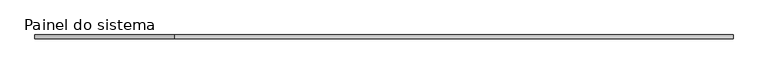
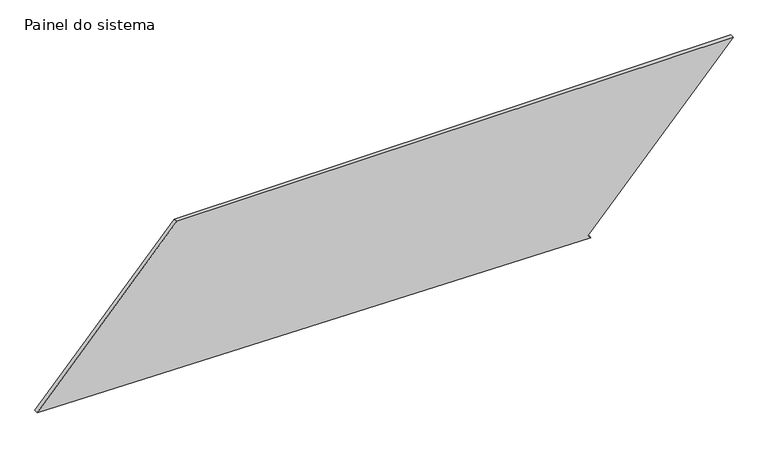
"""IFC4 building model written with IfcOpenShell, lengths in millimetres: plate geometry, Painel do sistema : Envidraçado."""

from ifc_helpers import new_model, si_unit, frame, origin, place, context, project, spatial, polyline, outline, extrude, source, transform, mapped, element, save


def painel_do_sistema_607a5ea9(model_context):
    return source(origin(), model_context, "Body", "SweptSolid", [
        extrude(outline(polyline([(0.0, 1274.6669561), (16.8339598, 1256.1840506), (1003.7131558, 2155.0191769), (1003.7131558, -1290.9067743), (54.9578968, -2155.0191769), (0.0, 1274.6669561)])), frame((0.0, 24.5, 0.0), z_axis=(0.0, 1.0, 0.0), x_axis=(0.0, 0.0, 1.0)), (0.0, 0.0, 1.0), 25.0),
    ])


if __name__ == "__main__":
    model = new_model("IFC4")
    model_context = context("Model", 3, world=origin())
    ifc_project = project(units=[si_unit("LENGTHUNIT", "METRE", prefix="MILLI")], contexts=[model_context])
    site = spatial("IfcSite", under=ifc_project)
    building = spatial("IfcBuilding", under=site)
    placement = place(None, origin())
    painel_do_sistema_shape = painel_do_sistema_607a5ea9(model_context)
    element("IfcPlate", 1, ObjectType="Painel do sistema : Envidraçado", at=placement, inside=building, context=model_context, shape_type="MappedRepresentation", body=[
        mapped(painel_do_sistema_shape, transform((0.0, 0.0, 0.0), x_axis=(1.0, 0.0, 0.0), y_axis=(0.0, 1.0, 0.0), z_axis=(0.0, 0.0, 1.0))),
    ])
    save(model, "model.ifc")

# Revit data of these elements
# Type "Painel do sistema : Envidraçado"
#   Construction Type Id = "GSP4R"
#   Analytic Construction = "Vidraça única Pilkington 1/8 pol"
#   Visual Light Transmittance = 0.9
#   Solar Heat Gain Coefficient = 0.86
#   Heat Transfer Coefficient (U) = 6.7069 W/(m²·K)
# Element 1 (IfcPlate, "Painel do sistema : Envidraçado")
#   Materials on its faces: "Vidro"
# Materials
#   "Vidro": class "Vidro", colour RGB 0 128 192, transparency 0.9, Description = "Vidro de sílica", Cost = 0
